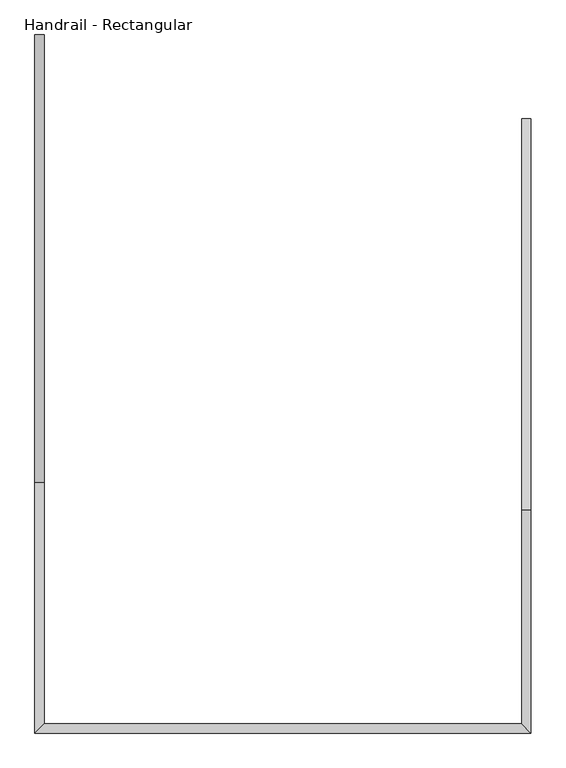
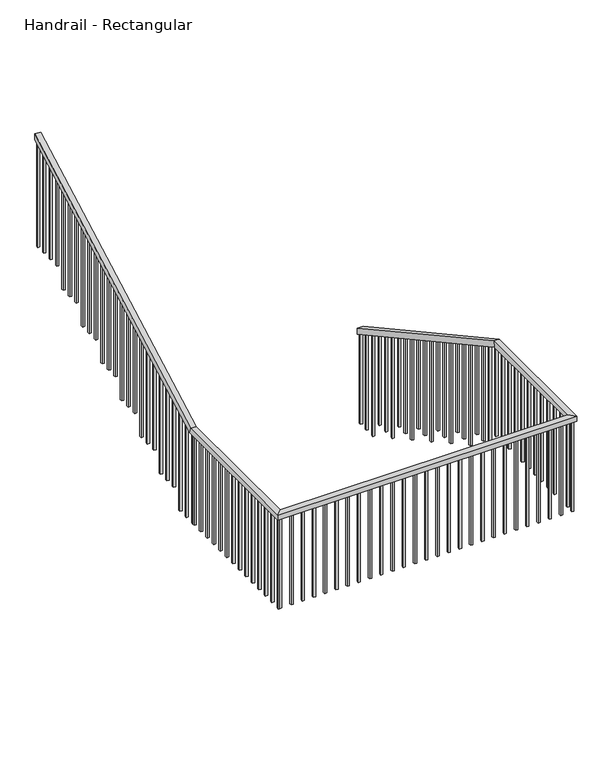
"""IFC4 building model written with IfcOpenShell, lengths in millimetres: railing geometry, Handrail - Rectangular."""

import ifcopenshell
import ifcopenshell.guid

model = None  # the IFC model being written
_history = None  # IfcOwnerHistory: only IFC2X3 demands one
_inside = {}  # id of a spatial element -> (the spatial element, [elements in it])
_under = {}  # id of a project, library or spatial element -> (it, [spatial elements below it])
_declared = {}  # id of a project -> (the project, [libraries it declares])
_typed = {}  # id of a type object -> (the type object, [elements of that type])
_made_of = {}  # id of a material, layer set ... -> (it, [elements and type objects made of it])


def new_model(schema):
    """Start an empty IFC model of exactly this schema.

    Asked for "IFC4X3", IfcOpenShell would pick the latest addendum, in which some entities
    have other attributes; the version numbers below select the first issue.
    IFC2X3 requires an IfcOwnerHistory on every rooted entity: one is made here for all.
    """
    global model, _history
    if schema == "IFC4X3":
        model = ifcopenshell.file(schema_version=(4, 3, 0, 0))
    else:
        model = ifcopenshell.file(schema=schema)
    _inside.clear()
    _under.clear()
    _declared.clear()
    _typed.clear()
    _made_of.clear()
    _history = None
    if model.schema == "IFC2X3":
        org = make("IfcOrganization", Name="unknown")
        user = make(
            "IfcPersonAndOrganization",
            ThePerson=make("IfcPerson", FamilyName="unknown"),
            TheOrganization=org,
        )
        app = make(
            "IfcApplication",
            ApplicationDeveloper=org,
            Version="unknown",
            ApplicationFullName="unknown",
            ApplicationIdentifier="unknown",
        )
        _history = make(
            "IfcOwnerHistory",
            OwningUser=user,
            OwningApplication=app,
            ChangeAction="ADDED",
            CreationDate=0,
        )
    return model


def make(cls, **values):
    """One entity of the class cls with the attributes given. An attribute that is None is left unset."""
    return model.create_entity(
        cls, **{name: value for name, value in values.items() if value is not None}
    )


def rooted(cls, **values):
    """An entity with a GlobalId (a new one), such as an element, a storey or a relation."""
    return make(cls, GlobalId=ifcopenshell.guid.new(), OwnerHistory=_history, **values)


def si_unit(unit_type, name, prefix=None):
    """IfcSIUnit, for example si_unit("LENGTHUNIT", "METRE", prefix="MILLI")."""
    return make("IfcSIUnit", UnitType=unit_type, Prefix=prefix, Name=name)


def assignment(units):
    """IfcUnitAssignment: the units of a project."""
    return None if units is None else make("IfcUnitAssignment", Units=units)


def point(xyz):
    """IfcCartesianPoint."""
    return None if xyz is None else make("IfcCartesianPoint", Coordinates=xyz)


def direction(xyz):
    """IfcDirection."""
    return None if xyz is None else make("IfcDirection", DirectionRatios=xyz)


def frame(location, z_axis=None, x_axis=None):
    """IfcAxis2Placement3D, a coordinate frame: its origin and axes. An axis left out is left unset."""
    return make(
        "IfcAxis2Placement3D",
        Location=point(location),
        Axis=direction(z_axis),
        RefDirection=direction(x_axis),
    )


def origin():
    """The frame at (0, 0, 0) with its axes left unset."""
    return frame((0.0, 0.0, 0.0))


def place(relative_to, where):
    """IfcLocalPlacement: puts the frame where relative to a parent placement (None: the world)."""
    return make(
        "IfcLocalPlacement", PlacementRelTo=relative_to, RelativePlacement=where
    )


def context(
    kind, dimensions, precision=None, world=None, true_north=None, identifier=None
):
    """IfcGeometricRepresentationContext, for example the 3D "Model" context."""
    return make(
        "IfcGeometricRepresentationContext",
        ContextIdentifier=identifier,
        ContextType=kind,
        CoordinateSpaceDimension=dimensions,
        Precision=precision,
        WorldCoordinateSystem=world,
        TrueNorth=true_north,
    )


def project(units=None, contexts=None):
    """IfcProject with its units and contexts."""
    return rooted(
        "IfcProject",
        Name="project",
        RepresentationContexts=contexts,
        UnitsInContext=assignment(units),
    )


def spatial(cls, under=None, at=None, **own):
    """A site, building, storey or space (cls), placed at a placement, below another one or the project."""
    s = rooted(cls, ObjectPlacement=at, **own)
    if under is not None:
        _under.setdefault(under.id(), (under, []))[1].append(s)
    return s


def polyline(points):
    """IfcPolyline through the points."""
    return make("IfcPolyline", Points=[point(p) for p in points])


def outline(outer, holes=None, kind="AREA"):
    """IfcArbitraryClosedProfileDef: a profile drawn as a closed curve; with holes, ...WithVoids."""
    if holes is None:
        return make("IfcArbitraryClosedProfileDef", ProfileType=kind, OuterCurve=outer)
    return make(
        "IfcArbitraryProfileDefWithVoids",
        ProfileType=kind,
        OuterCurve=outer,
        InnerCurves=holes,
    )


def extrude(swept, where, along, depth):
    """IfcExtrudedAreaSolid: the profile swept, set in the frame where, extruded along a direction by depth."""
    return make(
        "IfcExtrudedAreaSolid",
        SweptArea=swept,
        Position=where,
        ExtrudedDirection=direction(along),
        Depth=depth,
    )


def faces_of(points, faces, orient=None, outer=None):
    """IfcFace entities. A face is a list of loops; a loop is a list of indices into points, from 0.

    orient and outer hold one flag for each loop. By default every Orientation is true, the
    first loop of a face is its IfcFaceOuterBound and the others are IfcFaceBound.
    """
    made = []
    for i, loops in enumerate(faces):
        bounds = []
        for j, loop in enumerate(loops):
            is_outer = j == 0 if outer is None else outer[i][j]
            bounds.append(
                make(
                    "IfcFaceOuterBound" if is_outer else "IfcFaceBound",
                    Bound=make("IfcPolyLoop", Polygon=[points[k] for k in loop]),
                    Orientation=True if orient is None else orient[i][j],
                )
            )
        made.append(make("IfcFace", Bounds=bounds))
    return made


def faceted_brep(points, faces, orient=None, outer=None, voids=None):
    """IfcFacetedBrep: a solid bounded by flat faces; with voids (closed shells), ...WithVoids."""
    shared = [point(p) for p in points]
    hull = make("IfcClosedShell", CfsFaces=faces_of(shared, faces, orient, outer))
    if voids is None:
        return make("IfcFacetedBrep", Outer=hull)
    return make(
        "IfcFacetedBrepWithVoids",
        Outer=hull,
        Voids=[
            make(cls, CfsFaces=faces_of(shared, fs, o, b)) for cls, fs, o, b in voids
        ],
    )


def shape(context_of_items, identifier, shape_type, items):
    """IfcShapeRepresentation: the items that make up one representation, for example the "Body"."""
    return make(
        "IfcShapeRepresentation",
        ContextOfItems=context_of_items,
        RepresentationIdentifier=identifier,
        RepresentationType=shape_type,
        Items=items,
    )


def source(mapping_origin, context_of_items, identifier, shape_type, items):
    """IfcRepresentationMap: a shape defined once, which mapped items show again and again."""
    return make(
        "IfcRepresentationMap",
        MappingOrigin=mapping_origin,
        MappedRepresentation=shape(context_of_items, identifier, shape_type, items),
    )


def transform(
    local_origin,
    x_axis=None,
    y_axis=None,
    z_axis=None,
    scale=None,
    scale2=None,
    scale3=None,
    uniform=True,
):
    """IfcCartesianTransformationOperator3D, or its non-uniform kind. x_axis, y_axis, z_axis: its Axis1, 2, 3."""
    if uniform:
        return make(
            "IfcCartesianTransformationOperator3D",
            Axis1=direction(x_axis),
            Axis2=direction(y_axis),
            LocalOrigin=point(local_origin),
            Scale=scale,
            Axis3=direction(z_axis),
        )
    return make(
        "IfcCartesianTransformationOperator3DnonUniform",
        Axis1=direction(x_axis),
        Axis2=direction(y_axis),
        LocalOrigin=point(local_origin),
        Scale=scale,
        Axis3=direction(z_axis),
        Scale2=scale2,
        Scale3=scale3,
    )


def mapped(mapping_source, mapping_target):
    """IfcMappedItem: shows the shape of a source again, moved by a transform."""
    return make(
        "IfcMappedItem", MappingSource=mapping_source, MappingTarget=mapping_target
    )


def made_of(thing, what):
    """Note that an element or type object is made of a material, layer set ...; save() writes the relation."""
    if what is not None:
        _made_of.setdefault(what.id(), (what, []))[1].append(thing)
    return thing


def element(
    cls,
    number,
    at=None,
    inside=None,
    cuts=None,
    type_object=None,
    material=None,
    context=None,
    identifier="Body",
    shape_type=None,
    held_by="IfcProductDefinitionShape",
    body=None,
    shapes=None,
    **own,
):
    """One element of the class cls, such as IfcWall. Its Tag is "e" and its number.

    at: its placement. inside: the storey or other place that contains it. cuts: it is an
    opening in that element (IfcRelVoidsElement). A single representation is given by context,
    identifier, shape_type and body (its items); several are given by shapes. held_by: the class
    of the entity that holds the representations. save() writes the other relations.
    """
    e = rooted(cls, Tag="e%d" % number, ObjectPlacement=at, **own)
    if body is not None:
        shapes = [shape(context, identifier, shape_type, body)]
    if shapes is not None:
        e.Representation = make(held_by, Representations=shapes)
    if inside is not None:
        _inside.setdefault(inside.id(), (inside, []))[1].append(e)
    if cuts is not None:
        rooted(
            "IfcRelVoidsElement", RelatingBuildingElement=cuts, RelatedOpeningElement=e
        )
    if type_object is not None:
        _typed.setdefault(type_object.id(), (type_object, []))[1].append(e)
    return made_of(e, material)


def aggregate(whole, parts):
    """IfcRelAggregates: a whole, such as a stair, and the parts it consists of."""
    return rooted("IfcRelAggregates", RelatingObject=whole, RelatedObjects=parts)


def save(model, path):
    """Write the relations noted so far, then the file.

    IfcRelAggregates (storeys below a building ...), IfcRelContainedInSpatialStructure (elements
    in a storey), IfcRelDefinesByType, IfcRelAssociatesMaterial and IfcRelDeclares: one each for
    every whole, place, type object, material and project.
    """
    for whole, parts in _under.values():
        aggregate(whole, parts)
    for where, things in _inside.values():
        rooted(
            "IfcRelContainedInSpatialStructure",
            RelatedElements=things,
            RelatingStructure=where,
        )
    for kind, things in _typed.values():
        rooted("IfcRelDefinesByType", RelatedObjects=things, RelatingType=kind)
    for what, things in _made_of.values():
        rooted("IfcRelAssociatesMaterial", RelatedObjects=things, RelatingMaterial=what)
    for by, libraries in _declared.values():
        rooted("IfcRelDeclares", RelatingContext=by, RelatedDefinitions=libraries)
    model.write(path)


def handrail_rectangular_cd72d91a(model_context):
    return source(origin(), model_context, "Body", "SolidModel", [
        faceted_brep([(-73285.35, 12185.65, 17490.1411765), (-73285.35, 12185.65, 17432.1885835), (-73336.15, 12185.65, 17432.1885835), (-73336.15, 12185.65, 17490.1411765), (-73285.35, 10052.05, 18661.5294118), (-73285.35, 10039.0220627, 18610.7294118), (-73336.15, 10039.0220627, 18610.7294118), (-73336.15, 10052.05, 18661.5294118), (-73285.35, 8839.2, 18661.5294118), (-73285.35, 8839.2, 18610.7294118), (-73336.15, 8890.0, 18610.7294118), (-73336.15, 8890.0, 18661.5294118), (-75990.45, 8839.2, 18661.5294118), (-75990.45, 8839.2, 18610.7294118), (-75939.65, 8890.0, 18610.7294118), (-75939.65, 8890.0, 18661.5294118), (-75990.45, 10204.45, 18661.5294118), (-75990.45, 10217.4779373, 18610.7294118), (-75939.65, 10217.4779373, 18610.7294118), (-75939.65, 10204.45, 18661.5294118), (-75990.45, 12642.85, 20000.2588235), (-75939.65, 12642.85, 20000.2588235), (-75939.65, 12642.85, 19942.3062305), (-75990.45, 12642.85, 19942.3062305)], [[[0, 1, 2, 3]], [[1, 0, 4, 5]], [[2, 1, 5, 6]], [[3, 2, 6, 7]], [[0, 3, 7, 4]], [[5, 4, 8, 9]], [[6, 5, 9, 10]], [[7, 6, 10, 11]], [[4, 7, 11, 8]], [[9, 8, 12, 13]], [[10, 9, 13, 14]], [[11, 10, 14, 15]], [[8, 11, 15, 12]], [[13, 12, 16, 17]], [[14, 13, 17, 18]], [[15, 14, 18, 19]], [[12, 15, 19, 16]], [[20, 21, 22, 23]], [[17, 16, 20, 23]], [[18, 17, 23, 22]], [[19, 18, 22, 21]], [[16, 19, 21, 20]]]),
        extrude(outline(polyline([(12550.775, 19891.7552501), (12550.775, 18918.5176471), (12531.725, 18918.5176471), (12531.725, 19881.2964266), (12550.775, 19891.7552501)])), frame((-75974.575, 0.0, 0.0), z_axis=(1.0, 0.0, 0.0), x_axis=(0.0, 1.0, 0.0)), (0.0, 0.0, 1.0), 19.05),
        extrude(outline(polyline([(12449.175, 19835.974858), (12449.175, 18918.5176471), (12430.125, 18918.5176471), (12430.125, 19825.5160344), (12449.175, 19835.974858)])), frame((-75974.575, 0.0, 0.0), z_axis=(1.0, 0.0, 0.0), x_axis=(0.0, 1.0, 0.0)), (0.0, 0.0, 1.0), 19.05),
        extrude(outline(polyline([(12347.575, 19780.1944658), (12347.575, 18918.5176471), (12328.525, 18918.5176471), (12328.525, 19769.7356423), (12347.575, 19780.1944658)])), frame((-75974.575, 0.0, 0.0), z_axis=(1.0, 0.0, 0.0), x_axis=(0.0, 1.0, 0.0)), (0.0, 0.0, 1.0), 19.05),
        extrude(outline(polyline([(12245.975, 19724.4140737), (12245.975, 18751.1764706), (12226.925, 18751.1764706), (12226.925, 19713.9552501), (12245.975, 19724.4140737)])), frame((-75974.575, 0.0, 0.0), z_axis=(1.0, 0.0, 0.0), x_axis=(0.0, 1.0, 0.0)), (0.0, 0.0, 1.0), 19.05),
        extrude(outline(polyline([(12144.375, 19668.6336815), (12144.375, 18751.1764706), (12125.325, 18751.1764706), (12125.325, 19658.174858), (12144.375, 19668.6336815)])), frame((-75974.575, 0.0, 0.0), z_axis=(1.0, 0.0, 0.0), x_axis=(0.0, 1.0, 0.0)), (0.0, 0.0, 1.0), 19.05),
        extrude(outline(polyline([(12042.775, 19612.8532893), (12042.775, 18751.1764706), (12023.725, 18751.1764706), (12023.725, 19602.3944658), (12042.775, 19612.8532893)])), frame((-75974.575, 0.0, 0.0), z_axis=(1.0, 0.0, 0.0), x_axis=(0.0, 1.0, 0.0)), (0.0, 0.0, 1.0), 19.05),
        extrude(outline(polyline([(11941.175, 19557.0728972), (11941.175, 18583.8352941), (11922.125, 18583.8352941), (11922.125, 19546.6140737), (11941.175, 19557.0728972)])), frame((-75974.575, 0.0, 0.0), z_axis=(1.0, 0.0, 0.0), x_axis=(0.0, 1.0, 0.0)), (0.0, 0.0, 1.0), 19.05),
        extrude(outline(polyline([(11839.575, 19501.292505), (11839.575, 18583.8352941), (11820.525, 18583.8352941), (11820.525, 19490.8336815), (11839.575, 19501.292505)])), frame((-75974.575, 0.0, 0.0), z_axis=(1.0, 0.0, 0.0), x_axis=(0.0, 1.0, 0.0)), (0.0, 0.0, 1.0), 19.05),
        extrude(outline(polyline([(11737.975, 19445.5121129), (11737.975, 18583.8352941), (11718.925, 18583.8352941), (11718.925, 19435.0532893), (11737.975, 19445.5121129)])), frame((-75974.575, 0.0, 0.0), z_axis=(1.0, 0.0, 0.0), x_axis=(0.0, 1.0, 0.0)), (0.0, 0.0, 1.0), 19.05),
        extrude(outline(polyline([(11636.375, 19389.7317207), (11636.375, 18416.4941176), (11617.325, 18416.4941176), (11617.325, 19379.2728972), (11636.375, 19389.7317207)])), frame((-75974.575, 0.0, 0.0), z_axis=(1.0, 0.0, 0.0), x_axis=(0.0, 1.0, 0.0)), (0.0, 0.0, 1.0), 19.05),
        extrude(outline(polyline([(11534.775, 19333.9513286), (11534.775, 18416.4941176), (11515.725, 18416.4941176), (11515.725, 19323.492505), (11534.775, 19333.9513286)])), frame((-75974.575, 0.0, 0.0), z_axis=(1.0, 0.0, 0.0), x_axis=(0.0, 1.0, 0.0)), (0.0, 0.0, 1.0), 19.05),
        extrude(outline(polyline([(11433.175, 19278.1709364), (11433.175, 18416.4941176), (11414.125, 18416.4941176), (11414.125, 19267.7121129), (11433.175, 19278.1709364)])), frame((-75974.575, 0.0, 0.0), z_axis=(1.0, 0.0, 0.0), x_axis=(0.0, 1.0, 0.0)), (0.0, 0.0, 1.0), 19.05),
        extrude(outline(polyline([(11331.575, 19222.3905442), (11331.575, 18249.1529412), (11312.525, 18249.1529412), (11312.525, 19211.9317207), (11331.575, 19222.3905442)])), frame((-75974.575, 0.0, 0.0), z_axis=(1.0, 0.0, 0.0), x_axis=(0.0, 1.0, 0.0)), (0.0, 0.0, 1.0), 19.05),
        extrude(outline(polyline([(11229.975, 19166.6101521), (11229.975, 18249.1529412), (11210.925, 18249.1529412), (11210.925, 19156.1513286), (11229.975, 19166.6101521)])), frame((-75974.575, 0.0, 0.0), z_axis=(1.0, 0.0, 0.0), x_axis=(0.0, 1.0, 0.0)), (0.0, 0.0, 1.0), 19.05),
        extrude(outline(polyline([(11128.375, 19110.8297599), (11128.375, 18249.1529412), (11109.325, 18249.1529412), (11109.325, 19100.3709364), (11128.375, 19110.8297599)])), frame((-75974.575, 0.0, 0.0), z_axis=(1.0, 0.0, 0.0), x_axis=(0.0, 1.0, 0.0)), (0.0, 0.0, 1.0), 19.05),
        extrude(outline(polyline([(11026.775, 19055.0493678), (11026.775, 18081.8117647), (11007.725, 18081.8117647), (11007.725, 19044.5905442), (11026.775, 19055.0493678)])), frame((-75974.575, 0.0, 0.0), z_axis=(1.0, 0.0, 0.0), x_axis=(0.0, 1.0, 0.0)), (0.0, 0.0, 1.0), 19.05),
        extrude(outline(polyline([(10925.175, 18999.2689756), (10925.175, 18081.8117647), (10906.125, 18081.8117647), (10906.125, 18988.8101521), (10925.175, 18999.2689756)])), frame((-75974.575, 0.0, 0.0), z_axis=(1.0, 0.0, 0.0), x_axis=(0.0, 1.0, 0.0)), (0.0, 0.0, 1.0), 19.05),
        extrude(outline(polyline([(10823.575, 18943.4885835), (10823.575, 18081.8117647), (10804.525, 18081.8117647), (10804.525, 18933.0297599), (10823.575, 18943.4885835)])), frame((-75974.575, 0.0, 0.0), z_axis=(1.0, 0.0, 0.0), x_axis=(0.0, 1.0, 0.0)), (0.0, 0.0, 1.0), 19.05),
        extrude(outline(polyline([(10721.975, 18887.7081913), (10721.975, 17914.4705882), (10702.925, 17914.4705882), (10702.925, 18877.2493678), (10721.975, 18887.7081913)])), frame((-75974.575, 0.0, 0.0), z_axis=(1.0, 0.0, 0.0), x_axis=(0.0, 1.0, 0.0)), (0.0, 0.0, 1.0), 19.05),
        extrude(outline(polyline([(10620.375, 18831.9277991), (10620.375, 17914.4705882), (10601.325, 17914.4705882), (10601.325, 18821.4689756), (10620.375, 18831.9277991)])), frame((-75974.575, 0.0, 0.0), z_axis=(1.0, 0.0, 0.0), x_axis=(0.0, 1.0, 0.0)), (0.0, 0.0, 1.0), 19.05),
        extrude(outline(polyline([(10518.775, 18776.147407), (10518.775, 17914.4705882), (10499.725, 17914.4705882), (10499.725, 18765.6885835), (10518.775, 18776.147407)])), frame((-75974.575, 0.0, 0.0), z_axis=(1.0, 0.0, 0.0), x_axis=(0.0, 1.0, 0.0)), (0.0, 0.0, 1.0), 19.05),
        extrude(outline(polyline([(10417.175, 18720.3670148), (10417.175, 17747.1294118), (10398.125, 17747.1294118), (10398.125, 18709.9081913), (10417.175, 18720.3670148)])), frame((-75974.575, 0.0, 0.0), z_axis=(1.0, 0.0, 0.0), x_axis=(0.0, 1.0, 0.0)), (0.0, 0.0, 1.0), 19.05),
        extrude(outline(polyline([(10315.575, 18664.5866227), (10315.575, 17747.1294118), (10296.525, 17747.1294118), (10296.525, 18654.1277991), (10315.575, 18664.5866227)])), frame((-75974.575, 0.0, 0.0), z_axis=(1.0, 0.0, 0.0), x_axis=(0.0, 1.0, 0.0)), (0.0, 0.0, 1.0), 19.05),
        extrude(outline(polyline([(-75974.575, 10175.875), (-75974.575, 10194.925), (-75955.525, 10194.925), (-75955.525, 10175.875), (-75974.575, 10175.875)])), frame((0.0, 0.0, 17747.1294118), z_axis=(0.0, 0.0, 1.0), x_axis=(1.0, 0.0, 0.0)), (0.0, 0.0, 1.0), 863.6),
        extrude(outline(polyline([(-75974.575, 10074.275), (-75974.575, 10093.325), (-75955.525, 10093.325), (-75955.525, 10074.275), (-75974.575, 10074.275)])), frame((0.0, 0.0, 17747.1294118), z_axis=(0.0, 0.0, 1.0), x_axis=(1.0, 0.0, 0.0)), (0.0, 0.0, 1.0), 863.6),
        extrude(outline(polyline([(-75974.575, 9972.675), (-75974.575, 9991.725), (-75955.525, 9991.725), (-75955.525, 9972.675), (-75974.575, 9972.675)])), frame((0.0, 0.0, 17747.1294118), z_axis=(0.0, 0.0, 1.0), x_axis=(1.0, 0.0, 0.0)), (0.0, 0.0, 1.0), 863.6),
        extrude(outline(polyline([(-75974.575, 9871.075), (-75974.575, 9890.125), (-75955.525, 9890.125), (-75955.525, 9871.075), (-75974.575, 9871.075)])), frame((0.0, 0.0, 17747.1294118), z_axis=(0.0, 0.0, 1.0), x_axis=(1.0, 0.0, 0.0)), (0.0, 0.0, 1.0), 863.6),
        extrude(outline(polyline([(-75974.575, 9769.475), (-75974.575, 9788.525), (-75955.525, 9788.525), (-75955.525, 9769.475), (-75974.575, 9769.475)])), frame((0.0, 0.0, 17747.1294118), z_axis=(0.0, 0.0, 1.0), x_axis=(1.0, 0.0, 0.0)), (0.0, 0.0, 1.0), 863.6),
        extrude(outline(polyline([(-75974.575, 9667.875), (-75974.575, 9686.925), (-75955.525, 9686.925), (-75955.525, 9667.875), (-75974.575, 9667.875)])), frame((0.0, 0.0, 17747.1294118), z_axis=(0.0, 0.0, 1.0), x_axis=(1.0, 0.0, 0.0)), (0.0, 0.0, 1.0), 863.6),
        extrude(outline(polyline([(-75974.575, 9566.275), (-75974.575, 9585.325), (-75955.525, 9585.325), (-75955.525, 9566.275), (-75974.575, 9566.275)])), frame((0.0, 0.0, 17747.1294118), z_axis=(0.0, 0.0, 1.0), x_axis=(1.0, 0.0, 0.0)), (0.0, 0.0, 1.0), 863.6),
        extrude(outline(polyline([(-75974.575, 9464.675), (-75974.575, 9483.725), (-75955.525, 9483.725), (-75955.525, 9464.675), (-75974.575, 9464.675)])), frame((0.0, 0.0, 17747.1294118), z_axis=(0.0, 0.0, 1.0), x_axis=(1.0, 0.0, 0.0)), (0.0, 0.0, 1.0), 863.6),
        extrude(outline(polyline([(-75974.575, 9363.075), (-75974.575, 9382.125), (-75955.525, 9382.125), (-75955.525, 9363.075), (-75974.575, 9363.075)])), frame((0.0, 0.0, 17747.1294118), z_axis=(0.0, 0.0, 1.0), x_axis=(1.0, 0.0, 0.0)), (0.0, 0.0, 1.0), 863.6),
        extrude(outline(polyline([(-75974.575, 9261.475), (-75974.575, 9280.525), (-75955.525, 9280.525), (-75955.525, 9261.475), (-75974.575, 9261.475)])), frame((0.0, 0.0, 17747.1294118), z_axis=(0.0, 0.0, 1.0), x_axis=(1.0, 0.0, 0.0)), (0.0, 0.0, 1.0), 863.6),
        extrude(outline(polyline([(-75974.575, 9159.875), (-75974.575, 9178.925), (-75955.525, 9178.925), (-75955.525, 9159.875), (-75974.575, 9159.875)])), frame((0.0, 0.0, 17747.1294118), z_axis=(0.0, 0.0, 1.0), x_axis=(1.0, 0.0, 0.0)), (0.0, 0.0, 1.0), 863.6),
        extrude(outline(polyline([(-75974.575, 9058.275), (-75974.575, 9077.325), (-75955.525, 9077.325), (-75955.525, 9058.275), (-75974.575, 9058.275)])), frame((0.0, 0.0, 17747.1294118), z_axis=(0.0, 0.0, 1.0), x_axis=(1.0, 0.0, 0.0)), (0.0, 0.0, 1.0), 863.6),
        extrude(outline(polyline([(-75974.575, 8956.675), (-75974.575, 8975.725), (-75955.525, 8975.725), (-75955.525, 8956.675), (-75974.575, 8956.675)])), frame((0.0, 0.0, 17747.1294118), z_axis=(0.0, 0.0, 1.0), x_axis=(1.0, 0.0, 0.0)), (0.0, 0.0, 1.0), 863.6),
        extrude(outline(polyline([(-75942.825, 8855.075), (-75961.875, 8855.075), (-75961.875, 8874.125), (-75942.825, 8874.125), (-75942.825, 8855.075)])), frame((0.0, 0.0, 17747.1294118), z_axis=(0.0, 0.0, 1.0), x_axis=(1.0, 0.0, 0.0)), (0.0, 0.0, 1.0), 863.6),
        extrude(outline(polyline([(-75841.225, 8855.075), (-75860.275, 8855.075), (-75860.275, 8874.125), (-75841.225, 8874.125), (-75841.225, 8855.075)])), frame((0.0, 0.0, 17747.1294118), z_axis=(0.0, 0.0, 1.0), x_axis=(1.0, 0.0, 0.0)), (0.0, 0.0, 1.0), 863.6),
        extrude(outline(polyline([(-75739.625, 8855.075), (-75758.675, 8855.075), (-75758.675, 8874.125), (-75739.625, 8874.125), (-75739.625, 8855.075)])), frame((0.0, 0.0, 17747.1294118), z_axis=(0.0, 0.0, 1.0), x_axis=(1.0, 0.0, 0.0)), (0.0, 0.0, 1.0), 863.6),
        extrude(outline(polyline([(-75638.025, 8855.075), (-75657.075, 8855.075), (-75657.075, 8874.125), (-75638.025, 8874.125), (-75638.025, 8855.075)])), frame((0.0, 0.0, 17747.1294118), z_axis=(0.0, 0.0, 1.0), x_axis=(1.0, 0.0, 0.0)), (0.0, 0.0, 1.0), 863.6),
        extrude(outline(polyline([(-75536.425, 8855.075), (-75555.475, 8855.075), (-75555.475, 8874.125), (-75536.425, 8874.125), (-75536.425, 8855.075)])), frame((0.0, 0.0, 17747.1294118), z_axis=(0.0, 0.0, 1.0), x_axis=(1.0, 0.0, 0.0)), (0.0, 0.0, 1.0), 863.6),
        extrude(outline(polyline([(-75434.825, 8855.075), (-75453.875, 8855.075), (-75453.875, 8874.125), (-75434.825, 8874.125), (-75434.825, 8855.075)])), frame((0.0, 0.0, 17747.1294118), z_axis=(0.0, 0.0, 1.0), x_axis=(1.0, 0.0, 0.0)), (0.0, 0.0, 1.0), 863.6),
        extrude(outline(polyline([(-75333.225, 8855.075), (-75352.275, 8855.075), (-75352.275, 8874.125), (-75333.225, 8874.125), (-75333.225, 8855.075)])), frame((0.0, 0.0, 17747.1294118), z_axis=(0.0, 0.0, 1.0), x_axis=(1.0, 0.0, 0.0)), (0.0, 0.0, 1.0), 863.6),
        extrude(outline(polyline([(-75231.625, 8855.075), (-75250.675, 8855.075), (-75250.675, 8874.125), (-75231.625, 8874.125), (-75231.625, 8855.075)])), frame((0.0, 0.0, 17747.1294118), z_axis=(0.0, 0.0, 1.0), x_axis=(1.0, 0.0, 0.0)), (0.0, 0.0, 1.0), 863.6),
        extrude(outline(polyline([(-75130.025, 8855.075), (-75149.075, 8855.075), (-75149.075, 8874.125), (-75130.025, 8874.125), (-75130.025, 8855.075)])), frame((0.0, 0.0, 17747.1294118), z_axis=(0.0, 0.0, 1.0), x_axis=(1.0, 0.0, 0.0)), (0.0, 0.0, 1.0), 863.6),
        extrude(outline(polyline([(-75028.425, 8855.075), (-75047.475, 8855.075), (-75047.475, 8874.125), (-75028.425, 8874.125), (-75028.425, 8855.075)])), frame((0.0, 0.0, 17747.1294118), z_axis=(0.0, 0.0, 1.0), x_axis=(1.0, 0.0, 0.0)), (0.0, 0.0, 1.0), 863.6),
        extrude(outline(polyline([(-74926.825, 8855.075), (-74945.875, 8855.075), (-74945.875, 8874.125), (-74926.825, 8874.125), (-74926.825, 8855.075)])), frame((0.0, 0.0, 17747.1294118), z_axis=(0.0, 0.0, 1.0), x_axis=(1.0, 0.0, 0.0)), (0.0, 0.0, 1.0), 863.6),
        extrude(outline(polyline([(-74825.225, 8855.075), (-74844.275, 8855.075), (-74844.275, 8874.125), (-74825.225, 8874.125), (-74825.225, 8855.075)])), frame((0.0, 0.0, 17747.1294118), z_axis=(0.0, 0.0, 1.0), x_axis=(1.0, 0.0, 0.0)), (0.0, 0.0, 1.0), 863.6),
        extrude(outline(polyline([(-74723.625, 8855.075), (-74742.675, 8855.075), (-74742.675, 8874.125), (-74723.625, 8874.125), (-74723.625, 8855.075)])), frame((0.0, 0.0, 17747.1294118), z_axis=(0.0, 0.0, 1.0), x_axis=(1.0, 0.0, 0.0)), (0.0, 0.0, 1.0), 863.6),
        extrude(outline(polyline([(-74622.025, 8855.075), (-74641.075, 8855.075), (-74641.075, 8874.125), (-74622.025, 8874.125), (-74622.025, 8855.075)])), frame((0.0, 0.0, 17747.1294118), z_axis=(0.0, 0.0, 1.0), x_axis=(1.0, 0.0, 0.0)), (0.0, 0.0, 1.0), 863.6),
        extrude(outline(polyline([(-74520.425, 8855.075), (-74539.475, 8855.075), (-74539.475, 8874.125), (-74520.425, 8874.125), (-74520.425, 8855.075)])), frame((0.0, 0.0, 17747.1294118), z_axis=(0.0, 0.0, 1.0), x_axis=(1.0, 0.0, 0.0)), (0.0, 0.0, 1.0), 863.6),
        extrude(outline(polyline([(-74418.825, 8855.075), (-74437.875, 8855.075), (-74437.875, 8874.125), (-74418.825, 8874.125), (-74418.825, 8855.075)])), frame((0.0, 0.0, 17747.1294118), z_axis=(0.0, 0.0, 1.0), x_axis=(1.0, 0.0, 0.0)), (0.0, 0.0, 1.0), 863.6),
        extrude(outline(polyline([(-74317.225, 8855.075), (-74336.275, 8855.075), (-74336.275, 8874.125), (-74317.225, 8874.125), (-74317.225, 8855.075)])), frame((0.0, 0.0, 17747.1294118), z_axis=(0.0, 0.0, 1.0), x_axis=(1.0, 0.0, 0.0)), (0.0, 0.0, 1.0), 863.6),
        extrude(outline(polyline([(-74215.625, 8855.075), (-74234.675, 8855.075), (-74234.675, 8874.125), (-74215.625, 8874.125), (-74215.625, 8855.075)])), frame((0.0, 0.0, 17747.1294118), z_axis=(0.0, 0.0, 1.0), x_axis=(1.0, 0.0, 0.0)), (0.0, 0.0, 1.0), 863.6),
        extrude(outline(polyline([(-74114.025, 8855.075), (-74133.075, 8855.075), (-74133.075, 8874.125), (-74114.025, 8874.125), (-74114.025, 8855.075)])), frame((0.0, 0.0, 17747.1294118), z_axis=(0.0, 0.0, 1.0), x_axis=(1.0, 0.0, 0.0)), (0.0, 0.0, 1.0), 863.6),
        extrude(outline(polyline([(-74012.425, 8855.075), (-74031.475, 8855.075), (-74031.475, 8874.125), (-74012.425, 8874.125), (-74012.425, 8855.075)])), frame((0.0, 0.0, 17747.1294118), z_axis=(0.0, 0.0, 1.0), x_axis=(1.0, 0.0, 0.0)), (0.0, 0.0, 1.0), 863.6),
        extrude(outline(polyline([(-73910.825, 8855.075), (-73929.875, 8855.075), (-73929.875, 8874.125), (-73910.825, 8874.125), (-73910.825, 8855.075)])), frame((0.0, 0.0, 17747.1294118), z_axis=(0.0, 0.0, 1.0), x_axis=(1.0, 0.0, 0.0)), (0.0, 0.0, 1.0), 863.6),
        extrude(outline(polyline([(-73809.225, 8855.075), (-73828.275, 8855.075), (-73828.275, 8874.125), (-73809.225, 8874.125), (-73809.225, 8855.075)])), frame((0.0, 0.0, 17747.1294118), z_axis=(0.0, 0.0, 1.0), x_axis=(1.0, 0.0, 0.0)), (0.0, 0.0, 1.0), 863.6),
        extrude(outline(polyline([(-73707.625, 8855.075), (-73726.675, 8855.075), (-73726.675, 8874.125), (-73707.625, 8874.125), (-73707.625, 8855.075)])), frame((0.0, 0.0, 17747.1294118), z_axis=(0.0, 0.0, 1.0), x_axis=(1.0, 0.0, 0.0)), (0.0, 0.0, 1.0), 863.6),
        extrude(outline(polyline([(-73606.025, 8855.075), (-73625.075, 8855.075), (-73625.075, 8874.125), (-73606.025, 8874.125), (-73606.025, 8855.075)])), frame((0.0, 0.0, 17747.1294118), z_axis=(0.0, 0.0, 1.0), x_axis=(1.0, 0.0, 0.0)), (0.0, 0.0, 1.0), 863.6),
        extrude(outline(polyline([(-73504.425, 8855.075), (-73523.475, 8855.075), (-73523.475, 8874.125), (-73504.425, 8874.125), (-73504.425, 8855.075)])), frame((0.0, 0.0, 17747.1294118), z_axis=(0.0, 0.0, 1.0), x_axis=(1.0, 0.0, 0.0)), (0.0, 0.0, 1.0), 863.6),
        extrude(outline(polyline([(-73402.825, 8855.075), (-73421.875, 8855.075), (-73421.875, 8874.125), (-73402.825, 8874.125), (-73402.825, 8855.075)])), frame((0.0, 0.0, 17747.1294118), z_axis=(0.0, 0.0, 1.0), x_axis=(1.0, 0.0, 0.0)), (0.0, 0.0, 1.0), 863.6),
        extrude(outline(polyline([(-73301.225, 8943.975), (-73301.225, 8924.925), (-73320.275, 8924.925), (-73320.275, 8943.975), (-73301.225, 8943.975)])), frame((0.0, 0.0, 17747.1294118), z_axis=(0.0, 0.0, 1.0), x_axis=(1.0, 0.0, 0.0)), (0.0, 0.0, 1.0), 863.6),
        extrude(outline(polyline([(-73301.225, 9045.575), (-73301.225, 9026.525), (-73320.275, 9026.525), (-73320.275, 9045.575), (-73301.225, 9045.575)])), frame((0.0, 0.0, 17747.1294118), z_axis=(0.0, 0.0, 1.0), x_axis=(1.0, 0.0, 0.0)), (0.0, 0.0, 1.0), 863.6),
        extrude(outline(polyline([(-73301.225, 9147.175), (-73301.225, 9128.125), (-73320.275, 9128.125), (-73320.275, 9147.175), (-73301.225, 9147.175)])), frame((0.0, 0.0, 17747.1294118), z_axis=(0.0, 0.0, 1.0), x_axis=(1.0, 0.0, 0.0)), (0.0, 0.0, 1.0), 863.6),
        extrude(outline(polyline([(-73301.225, 9248.775), (-73301.225, 9229.725), (-73320.275, 9229.725), (-73320.275, 9248.775), (-73301.225, 9248.775)])), frame((0.0, 0.0, 17747.1294118), z_axis=(0.0, 0.0, 1.0), x_axis=(1.0, 0.0, 0.0)), (0.0, 0.0, 1.0), 863.6),
        extrude(outline(polyline([(-73301.225, 9350.375), (-73301.225, 9331.325), (-73320.275, 9331.325), (-73320.275, 9350.375), (-73301.225, 9350.375)])), frame((0.0, 0.0, 17747.1294118), z_axis=(0.0, 0.0, 1.0), x_axis=(1.0, 0.0, 0.0)), (0.0, 0.0, 1.0), 863.6),
        extrude(outline(polyline([(-73301.225, 9451.975), (-73301.225, 9432.925), (-73320.275, 9432.925), (-73320.275, 9451.975), (-73301.225, 9451.975)])), frame((0.0, 0.0, 17747.1294118), z_axis=(0.0, 0.0, 1.0), x_axis=(1.0, 0.0, 0.0)), (0.0, 0.0, 1.0), 863.6),
        extrude(outline(polyline([(-73301.225, 9553.575), (-73301.225, 9534.525), (-73320.275, 9534.525), (-73320.275, 9553.575), (-73301.225, 9553.575)])), frame((0.0, 0.0, 17747.1294118), z_axis=(0.0, 0.0, 1.0), x_axis=(1.0, 0.0, 0.0)), (0.0, 0.0, 1.0), 863.6),
        extrude(outline(polyline([(-73301.225, 9655.175), (-73301.225, 9636.125), (-73320.275, 9636.125), (-73320.275, 9655.175), (-73301.225, 9655.175)])), frame((0.0, 0.0, 17747.1294118), z_axis=(0.0, 0.0, 1.0), x_axis=(1.0, 0.0, 0.0)), (0.0, 0.0, 1.0), 863.6),
        extrude(outline(polyline([(-73301.225, 9756.775), (-73301.225, 9737.725), (-73320.275, 9737.725), (-73320.275, 9756.775), (-73301.225, 9756.775)])), frame((0.0, 0.0, 17747.1294118), z_axis=(0.0, 0.0, 1.0), x_axis=(1.0, 0.0, 0.0)), (0.0, 0.0, 1.0), 863.6),
        extrude(outline(polyline([(-73301.225, 9858.375), (-73301.225, 9839.325), (-73320.275, 9839.325), (-73320.275, 9858.375), (-73301.225, 9858.375)])), frame((0.0, 0.0, 17747.1294118), z_axis=(0.0, 0.0, 1.0), x_axis=(1.0, 0.0, 0.0)), (0.0, 0.0, 1.0), 863.6),
        extrude(outline(polyline([(-73301.225, 9959.975), (-73301.225, 9940.925), (-73320.275, 9940.925), (-73320.275, 9959.975), (-73301.225, 9959.975)])), frame((0.0, 0.0, 17747.1294118), z_axis=(0.0, 0.0, 1.0), x_axis=(1.0, 0.0, 0.0)), (0.0, 0.0, 1.0), 863.6),
        extrude(outline(polyline([(10163.175, 18542.5670148), (10163.175, 17579.7882353), (10144.125, 17579.7882353), (10144.125, 18553.0258384), (10163.175, 18542.5670148)])), frame((-73320.275, 0.0, 0.0), z_axis=(1.0, 0.0, 0.0), x_axis=(0.0, 1.0, 0.0)), (0.0, 0.0, 1.0), 19.05),
        extrude(outline(polyline([(10264.775, 18486.7866227), (10264.775, 17579.7882353), (10245.725, 17579.7882353), (10245.725, 18497.2454462), (10264.775, 18486.7866227)])), frame((-73320.275, 0.0, 0.0), z_axis=(1.0, 0.0, 0.0), x_axis=(0.0, 1.0, 0.0)), (0.0, 0.0, 1.0), 19.05),
        extrude(outline(polyline([(10366.375, 18431.0062305), (10366.375, 17579.7882353), (10347.325, 17579.7882353), (10347.325, 18441.465054), (10366.375, 18431.0062305)])), frame((-73320.275, 0.0, 0.0), z_axis=(1.0, 0.0, 0.0), x_axis=(0.0, 1.0, 0.0)), (0.0, 0.0, 1.0), 19.05),
        extrude(outline(polyline([(10467.975, 18375.2258384), (10467.975, 17412.4470588), (10448.925, 17412.4470588), (10448.925, 18385.6846619), (10467.975, 18375.2258384)])), frame((-73320.275, 0.0, 0.0), z_axis=(1.0, 0.0, 0.0), x_axis=(0.0, 1.0, 0.0)), (0.0, 0.0, 1.0), 19.05),
        extrude(outline(polyline([(10569.575, 18319.4454462), (10569.575, 17412.4470588), (10550.525, 17412.4470588), (10550.525, 18329.9042697), (10569.575, 18319.4454462)])), frame((-73320.275, 0.0, 0.0), z_axis=(1.0, 0.0, 0.0), x_axis=(0.0, 1.0, 0.0)), (0.0, 0.0, 1.0), 19.05),
        extrude(outline(polyline([(10671.175, 18263.665054), (10671.175, 17412.4470588), (10652.125, 17412.4470588), (10652.125, 18274.1238776), (10671.175, 18263.665054)])), frame((-73320.275, 0.0, 0.0), z_axis=(1.0, 0.0, 0.0), x_axis=(0.0, 1.0, 0.0)), (0.0, 0.0, 1.0), 19.05),
        extrude(outline(polyline([(10772.775, 18207.8846619), (10772.775, 17245.1058824), (10753.725, 17245.1058824), (10753.725, 18218.3434854), (10772.775, 18207.8846619)])), frame((-73320.275, 0.0, 0.0), z_axis=(1.0, 0.0, 0.0), x_axis=(0.0, 1.0, 0.0)), (0.0, 0.0, 1.0), 19.05),
        extrude(outline(polyline([(10874.375, 18152.1042697), (10874.375, 17245.1058824), (10855.325, 17245.1058824), (10855.325, 18162.5630933), (10874.375, 18152.1042697)])), frame((-73320.275, 0.0, 0.0), z_axis=(1.0, 0.0, 0.0), x_axis=(0.0, 1.0, 0.0)), (0.0, 0.0, 1.0), 19.05),
        extrude(outline(polyline([(10975.975, 18096.3238776), (10975.975, 17245.1058824), (10956.925, 17245.1058824), (10956.925, 18106.7827011), (10975.975, 18096.3238776)])), frame((-73320.275, 0.0, 0.0), z_axis=(1.0, 0.0, 0.0), x_axis=(0.0, 1.0, 0.0)), (0.0, 0.0, 1.0), 19.05),
        extrude(outline(polyline([(11077.575, 18040.5434854), (11077.575, 17077.7647059), (11058.525, 17077.7647059), (11058.525, 18051.0023089), (11077.575, 18040.5434854)])), frame((-73320.275, 0.0, 0.0), z_axis=(1.0, 0.0, 0.0), x_axis=(0.0, 1.0, 0.0)), (0.0, 0.0, 1.0), 19.05),
        extrude(outline(polyline([(11179.175, 17984.7630933), (11179.175, 17077.7647059), (11160.125, 17077.7647059), (11160.125, 17995.2219168), (11179.175, 17984.7630933)])), frame((-73320.275, 0.0, 0.0), z_axis=(1.0, 0.0, 0.0), x_axis=(0.0, 1.0, 0.0)), (0.0, 0.0, 1.0), 19.05),
        extrude(outline(polyline([(11280.775, 17928.9827011), (11280.775, 17077.7647059), (11261.725, 17077.7647059), (11261.725, 17939.4415246), (11280.775, 17928.9827011)])), frame((-73320.275, 0.0, 0.0), z_axis=(1.0, 0.0, 0.0), x_axis=(0.0, 1.0, 0.0)), (0.0, 0.0, 1.0), 19.05),
        extrude(outline(polyline([(11382.375, 17873.2023089), (11382.375, 16910.4235294), (11363.325, 16910.4235294), (11363.325, 17883.6611325), (11382.375, 17873.2023089)])), frame((-73320.275, 0.0, 0.0), z_axis=(1.0, 0.0, 0.0), x_axis=(0.0, 1.0, 0.0)), (0.0, 0.0, 1.0), 19.05),
        extrude(outline(polyline([(11483.975, 17817.4219168), (11483.975, 16910.4235294), (11464.925, 16910.4235294), (11464.925, 17827.8807403), (11483.975, 17817.4219168)])), frame((-73320.275, 0.0, 0.0), z_axis=(1.0, 0.0, 0.0), x_axis=(0.0, 1.0, 0.0)), (0.0, 0.0, 1.0), 19.05),
        extrude(outline(polyline([(11585.575, 17761.6415246), (11585.575, 16910.4235294), (11566.525, 16910.4235294), (11566.525, 17772.1003482), (11585.575, 17761.6415246)])), frame((-73320.275, 0.0, 0.0), z_axis=(1.0, 0.0, 0.0), x_axis=(0.0, 1.0, 0.0)), (0.0, 0.0, 1.0), 19.05),
        extrude(outline(polyline([(11687.175, 17705.8611325), (11687.175, 16743.0823529), (11668.125, 16743.0823529), (11668.125, 17716.319956), (11687.175, 17705.8611325)])), frame((-73320.275, 0.0, 0.0), z_axis=(1.0, 0.0, 0.0), x_axis=(0.0, 1.0, 0.0)), (0.0, 0.0, 1.0), 19.05),
        extrude(outline(polyline([(11788.775, 17650.0807403), (11788.775, 16743.0823529), (11769.725, 16743.0823529), (11769.725, 17660.5395638), (11788.775, 17650.0807403)])), frame((-73320.275, 0.0, 0.0), z_axis=(1.0, 0.0, 0.0), x_axis=(0.0, 1.0, 0.0)), (0.0, 0.0, 1.0), 19.05),
        extrude(outline(polyline([(11890.375, 17594.3003482), (11890.375, 16743.0823529), (11871.325, 16743.0823529), (11871.325, 17604.7591717), (11890.375, 17594.3003482)])), frame((-73320.275, 0.0, 0.0), z_axis=(1.0, 0.0, 0.0), x_axis=(0.0, 1.0, 0.0)), (0.0, 0.0, 1.0), 19.05),
        extrude(outline(polyline([(11991.975, 17538.519956), (11991.975, 16575.7411765), (11972.925, 16575.7411765), (11972.925, 17548.9787795), (11991.975, 17538.519956)])), frame((-73320.275, 0.0, 0.0), z_axis=(1.0, 0.0, 0.0), x_axis=(0.0, 1.0, 0.0)), (0.0, 0.0, 1.0), 19.05),
        extrude(outline(polyline([(12093.575, 17482.7395638), (12093.575, 16575.7411765), (12074.525, 16575.7411765), (12074.525, 17493.1983874), (12093.575, 17482.7395638)])), frame((-73320.275, 0.0, 0.0), z_axis=(1.0, 0.0, 0.0), x_axis=(0.0, 1.0, 0.0)), (0.0, 0.0, 1.0), 19.05),
        extrude(outline(polyline([(-75974.575, 10194.925), (-75974.575, 10213.975), (-75955.525, 10213.975), (-75955.525, 10194.925), (-75974.575, 10194.925)])), frame((0.0, 0.0, 17747.1294118), z_axis=(0.0, 0.0, 1.0), x_axis=(1.0, 0.0, 0.0)), (0.0, 0.0, 1.0), 863.6),
        extrude(outline(polyline([(-75955.525, 8855.075), (-75974.575, 8855.075), (-75974.575, 8874.125), (-75955.525, 8874.125), (-75955.525, 8855.075)])), frame((0.0, 0.0, 17747.1294118), z_axis=(0.0, 0.0, 1.0), x_axis=(1.0, 0.0, 0.0)), (0.0, 0.0, 1.0), 863.6),
        extrude(outline(polyline([(-73301.225, 8874.125), (-73301.225, 8855.075), (-73320.275, 8855.075), (-73320.275, 8874.125), (-73301.225, 8874.125)])), frame((0.0, 0.0, 17747.1294118), z_axis=(0.0, 0.0, 1.0), x_axis=(1.0, 0.0, 0.0)), (0.0, 0.0, 1.0), 863.6),
        extrude(outline(polyline([(10061.575, 18598.347407), (10061.575, 17747.1294118), (10042.525, 17747.1294118), (10042.525, 18608.8062305), (10061.575, 18598.347407)])), frame((-73320.275, 0.0, 0.0), z_axis=(1.0, 0.0, 0.0), x_axis=(0.0, 1.0, 0.0)), (0.0, 0.0, 1.0), 19.05),
        extrude(outline(polyline([(12642.85, 19942.3062305), (12642.85, 18918.5176471), (12623.8, 18918.5176471), (12623.8, 19931.847407), (12642.85, 19942.3062305)])), frame((-75974.575, 0.0, 0.0), z_axis=(1.0, 0.0, 0.0), x_axis=(0.0, 1.0, 0.0)), (0.0, 0.0, 1.0), 19.05),
        extrude(outline(polyline([(12185.65, 17432.1885835), (12185.65, 16575.7411765), (12166.6, 16575.7411765), (12166.6, 17442.647407), (12185.65, 17432.1885835)])), frame((-73320.275, 0.0, 0.0), z_axis=(1.0, 0.0, 0.0), x_axis=(0.0, 1.0, 0.0)), (0.0, 0.0, 1.0), 19.05),
    ])


if __name__ == "__main__":
    model = new_model("IFC4")
    model_context = context("Model", 3, world=origin())
    ifc_project = project(units=[si_unit("LENGTHUNIT", "METRE", prefix="MILLI")], contexts=[model_context])
    site = spatial("IfcSite", under=ifc_project)
    building = spatial("IfcBuilding", under=site)
    placement = place(None, origin())
    handrail_rectangular_shape = handrail_rectangular_cd72d91a(model_context)
    element("IfcRailing", 1, ObjectType="Handrail - Rectangular", at=placement, inside=building, context=model_context, shape_type="MappedRepresentation", body=[
        mapped(handrail_rectangular_shape, transform((0.0, 0.0, 0.0), x_axis=(1.0, 0.0, 0.0), y_axis=(0.0, 1.0, 0.0), z_axis=(0.0, 0.0, 1.0))),
    ])
    save(model, "model.ifc")
